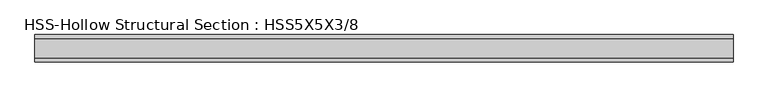
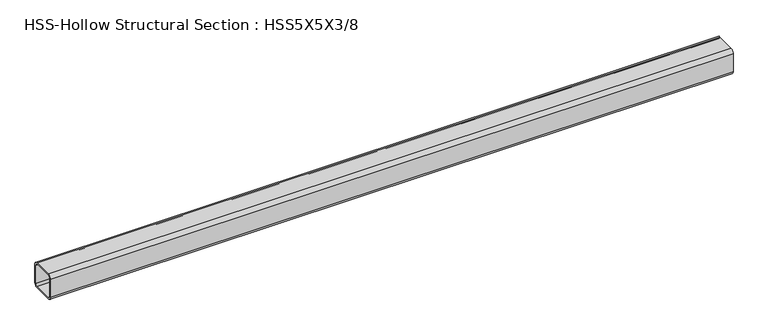
"""IFC4 building model written with IfcOpenShell, lengths in millimetres: member geometry, HSS-Hollow Structural Section : HSS5X5X3/8."""

from ifc_helpers import new_model, si_unit, point, frame, frame_2d, origin, place, context, project, spatial, polyline, circle_curve, trimmed, segment, composite_curve, outline, extrude, source, transform, mapped, element, save


def hss_hollow_structural_section_hss5x5x3_8_3030ebb5(model_context):
    return source(origin(), model_context, "Body", "SweptSolid", [
        extrude(outline(composite_curve([segment(polyline([(63.5, 45.7708), (63.5, -45.7708)]), True, "CONTINUOUS"), segment(trimmed(circle_curve(frame_2d((45.7708, -45.7708)), 17.7292), [point((63.5, -45.7708))], [point((45.7708, -63.5))], False, "CARTESIAN"), True, "CONTINUOUS"), segment(polyline([(45.7708, -63.5), (-45.7708, -63.5)]), True, "CONTINUOUS"), segment(trimmed(circle_curve(frame_2d((-45.7708, -45.7708)), 17.7292), [point((-45.7708, -63.5))], [point((-63.5, -45.7708))], False, "CARTESIAN"), True, "CONTINUOUS"), segment(polyline([(-63.5, -45.7708), (-63.5, 45.7708)]), True, "CONTINUOUS"), segment(trimmed(circle_curve(frame_2d((-45.7708, 45.7708)), 17.7292), [point((-63.5, 45.7708))], [point((-45.7708, 63.5))], False, "CARTESIAN"), True, "CONTINUOUS"), segment(polyline([(-45.7708, 63.5), (45.7708, 63.5)]), True, "CONTINUOUS"), segment(trimmed(circle_curve(frame_2d((45.7708, 45.7708)), 17.7292), [point((45.7708, 63.5))], [point((63.5, 45.7708))], False, "CARTESIAN"), True, "CONTINUOUS")], self_intersect=False), holes=[composite_curve([segment(trimmed(circle_curve(frame_2d((-45.7708, 45.7708)), 8.8646), [point((-45.7708, 54.6354))], [point((-54.6354, 45.7708))], True, "CARTESIAN"), True, "CONTINUOUS"), segment(polyline([(-54.6354, 45.7708), (-54.6354, -45.7708)]), True, "CONTINUOUS"), segment(trimmed(circle_curve(frame_2d((-45.7708, -45.7708)), 8.8646), [point((-54.6354, -45.7708))], [point((-45.7708, -54.6354))], True, "CARTESIAN"), True, "CONTINUOUS"), segment(polyline([(-45.7708, -54.6354), (45.7708, -54.6354)]), True, "CONTINUOUS"), segment(trimmed(circle_curve(frame_2d((45.7708, -45.7708)), 8.8646), [point((45.7708, -54.6354))], [point((54.6354, -45.7708))], True, "CARTESIAN"), True, "CONTINUOUS"), segment(polyline([(54.6354, -45.7708), (54.6354, 45.7708)]), True, "CONTINUOUS"), segment(trimmed(circle_curve(frame_2d((45.7708, 45.7708)), 8.8646), [point((54.6354, 45.7708))], [point((45.7708, 54.6354))], True, "CARTESIAN"), True, "CONTINUOUS"), segment(polyline([(45.7708, 54.6354), (-45.7708, 54.6354)]), True, "CONTINUOUS")], self_intersect=False)]), frame((-1560.8988968, 0.0, 0.0), z_axis=(1.0, 0.0, 0.0), x_axis=(0.0, 1.0, 0.0)), (0.0, 0.0, 1.0), 3260.100264),
    ])


if __name__ == "__main__":
    model = new_model("IFC4")
    model_context = context("Model", 3, world=origin())
    ifc_project = project(units=[si_unit("LENGTHUNIT", "METRE", prefix="MILLI")], contexts=[model_context])
    site = spatial("IfcSite", under=ifc_project)
    building = spatial("IfcBuilding", under=site)
    placement = place(None, origin())
    hss_hollow_structural_section_hss5x5x3_8_shape = hss_hollow_structural_section_hss5x5x3_8_3030ebb5(model_context)
    element("IfcMember", 1, ObjectType="HSS-Hollow Structural Section : HSS5X5X3/8", at=placement, inside=building, context=model_context, shape_type="MappedRepresentation", body=[
        mapped(hss_hollow_structural_section_hss5x5x3_8_shape, transform((0.0, 0.0, 0.0), x_axis=(1.0, 0.0, 0.0), y_axis=(0.0, 1.0, 0.0), z_axis=(0.0, 0.0, 1.0))),
    ])
    save(model, "model.ifc")

# Revit data of these elements
# Type "HSS-Hollow Structural Section : HSS5X5X3/8"
#   Assembly Code = "B10"
#   Shape = "Square"
#   W = 22.3
#   Ht = 0' - 5"
#   Length [instance default] = 5' - 0"
#   b = 0' - 5"
#   kr = 0' - 0.698"
#   t = 0' - 0.349"
#   A = 0.0429167 SF
#   Structural Material [instance default] = Steel ASTM A500, Grade B, Rectangular and Square
# Element 1 (IfcMember, "HSS-Hollow Structural Section : HSS5X5X3/8")
#   Materials on its faces: "Steel ASTM A500, Grade B, Rectangular and Square"
# Materials
#   "Steel ASTM A500, Grade B, Rectangular and Square": class "Metal", colour RGB 199 199 199, transparency 0, Description = "Carbon steel", Cost = 0
